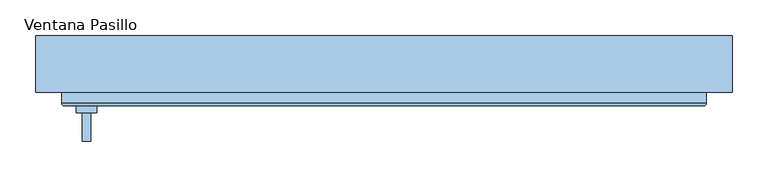
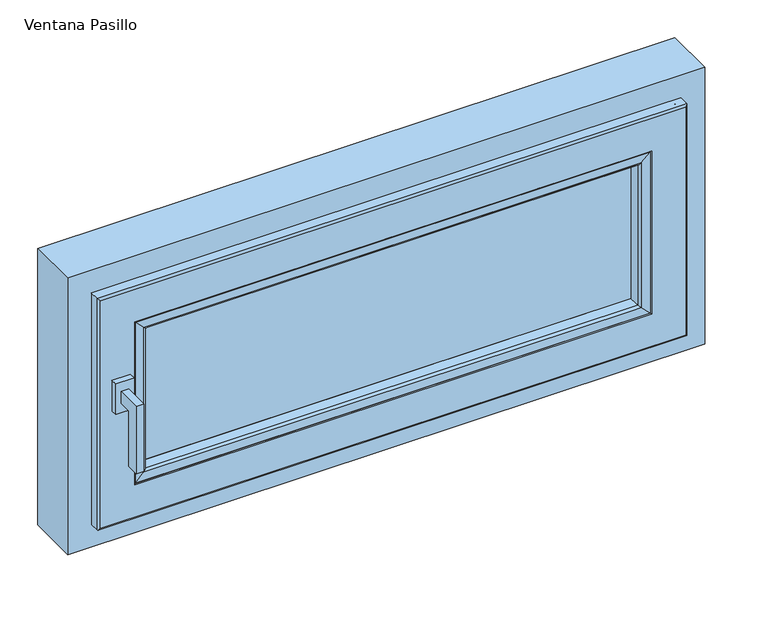
"""IFC4 building model written with IfcOpenShell, lengths in millimetres: window geometry, 2019_ES_Ventana_Replus_re80pvc301_10100_1-Hoja : Ventana Pasillo."""

from ifc_helpers import new_model, si_unit, frame, origin, place, context, project, spatial, polyline, ellipse_curve, outline, extrude, source, transform, mapped, element, save
from ifc_brep_helpers import plane_surface, cylinder_surface, advanced_brep


def ventana_pasillo_7f72e0b0(model_context):
    return source(origin(), model_context, "Body", "SolidModel", [
        extrude(outline(polyline([(-78.4999991, 1070.0), (-78.4999991, 1050.0), (-98.4999991, 1050.0), (-98.4999991, 960.0), (-118.4999991, 960.0), (-118.4999991, 1070.0), (-78.4999991, 1070.0)])), frame((-424.1999993, 0.0, 0.0), z_axis=(1.0, 0.0, 0.0), x_axis=(0.0, 1.0, 0.0)), (0.0, 0.0, 1.0), 12.0),
        extrude(outline(polyline([(-403.9687607, -78.4999991), (-432.4312378, -78.4999991), (-432.4312378, -68.4999991), (-403.9687607, -68.4999991), (-403.9687607, -78.4999991)])), frame((0.0, 0.0, 1035.217127), z_axis=(0.0, 0.0, 1.0), x_axis=(1.0, 0.0, 0.0)), (0.0, 0.0, 1.0), 49.565746),
        extrude(outline(polyline([(1157.2, 387.1999993), (1157.2, -387.1999993), (909.8, -387.1999993), (909.8, 387.1999993), (1157.2, 387.1999993)]), holes=[polyline([(917.8, 379.1999993), (917.8, -379.1999993), (1149.2, -379.1999993), (1149.2, 379.1999993), (917.8, 379.1999993)])]), frame((0.0, -26.9999999, 0.0), z_axis=(0.0, 1.0, 0.0), x_axis=(0.0, 0.0, 1.0)), (0.0, 0.0, 1.0), 16.0),
        extrude(outline(polyline([(1157.1868066, 387.1868058), (1157.1868066, -387.1868058), (909.8131934, -387.1868058), (909.8131934, 387.1868058), (1157.1868066, 387.1868058)]), holes=[polyline([(917.8, 379.1999993), (917.8, -379.1999993), (1149.2, -379.1999993), (1149.2, 379.1999993), (917.8, 379.1999993)])]), frame((0.0, -47.0000001, 0.0), z_axis=(0.0, 1.0, 0.0), x_axis=(0.0, 0.0, 1.0)), (0.0, 0.0, 1.0), 16.0),
        extrude(outline(polyline([(387.1999993, -6.9999997), (387.1999993, -10.9999999), (-387.1999993, -10.9999999), (-387.1999993, -6.9999997), (387.1999993, -6.9999997)])), frame((0.0, 0.0, 903.7946451), z_axis=(0.0, 0.0, 1.0), x_axis=(1.0, 0.0, 0.0)), (0.0, 0.0, 1.0), 259.4053549),
        extrude(outline(polyline([(387.1999993, -26.9999999), (387.1999993, -31.0000001), (-387.1999993, -31.0000001), (-387.1999993, -26.9999999), (387.1999993, -26.9999999)])), frame((0.0, 0.0, 903.7946451), z_axis=(0.0, 0.0, 1.0), x_axis=(1.0, 0.0, 0.0)), (0.0, 0.0, 1.0), 259.4053549),
        extrude(outline(polyline([(387.1999993, -47.0000001), (387.1999993, -51.0000003), (-387.1999993, -51.0000003), (-387.1999993, -47.0000001), (387.1999993, -47.0000001)])), frame((0.0, 0.0, 903.7946451), z_axis=(0.0, 0.0, 1.0), x_axis=(1.0, 0.0, 0.0)), (0.0, 0.0, 1.0), 259.4053549),
        advanced_brep(
        [(377.2913171, 9.2764571, 1147.2913178), (380.1890946, 11.5, 1150.1890953), (380.1890946, 11.5, 919.8109047), (377.2913171, 9.2764571, 922.7086822), (420.1999993, 11.5, 879.8), (-420.1999993, 11.5, 879.8), (-420.1999993, 11.5, 1190.2), (420.1999993, 11.5, 1190.2), (-380.1890946, 11.5, 1150.1890953), (-380.1890946, 11.5, 919.8109047), (-377.2913171, 9.2764571, 922.7086822), (374.1757968, -2.3508228, 1144.1757976), (374.1757968, -2.3508228, 925.8242024), (-374.1757968, -2.3508228, 925.8242024), (374.6739305, -3.0000033, 1144.6739313), (374.6739305, -3.0000033, 925.3260687), (-374.6739305, -3.0000033, 925.3260687), (381.1999993, -3.0000033, 1151.2), (-381.1999993, -3.0000033, 1151.2), (-381.1999993, -3.0000033, 918.8), (381.1999993, -3.0000033, 918.8), (-374.6739305, -3.0000033, 1144.6739313), (381.1999993, -6.9999997, 1151.2), (381.1999993, -6.9999997, 918.8), (-381.1999993, -6.9999997, 918.8), (401.8162192, -6.9999997, 1171.8162199), (-401.8162192, -6.9999997, 1171.8162199), (-401.8162192, -6.9999997, 898.1837801), (401.8162192, -6.9999997, 898.1837801), (-381.1999993, -6.9999997, 1151.2), (399.1999993, -25.6153717, 1169.2), (399.1999993, -25.6153717, 900.8), (-399.1999993, -25.6153717, 900.8), (399.1999993, -56.4999995, 1169.2), (399.1999993, -56.4999995, 900.8), (-399.1999993, -56.4999995, 900.8), (-399.1999993, -56.4999995, 1169.2), (387.1999993, -56.4999995, 1157.2), (-387.1999993, -56.4999995, 1157.2), (-387.1999993, -56.4999995, 912.8), (387.1999993, -56.4999995, 912.8), (387.1999993, -51.0000003, 1157.2), (387.1999993, -51.0000003, 912.8), (-387.1999993, -51.0000003, 912.8), (-387.1999993, -51.0000003, 1157.2), (376.007687, -51.0000003, 1146.0076877), (-376.007687, -51.0000003, 1146.0076877), (-376.007687, -51.0000003, 923.9923123), (376.007687, -51.0000003, 923.9923123), (375.4940999, -51.6693201, 1145.4941006), (375.4940999, -51.6693201, 924.5058994), (-375.4940999, -51.6693201, 924.5058994), (378.8993918, -64.3780426, 1148.8993925), (378.8993918, -64.3780426, 921.1006075), (-378.8993918, -64.3780426, 921.1006075), (382.6234971, -67.3403297, 1152.6234978), (382.6234971, -67.3403297, 917.3765022), (-382.6234971, -67.3403297, 917.3765022), (395.6488427, -67.7951848, 1165.6488434), (395.6488427, -67.7951848, 904.3511566), (-395.6488427, -67.7951848, 904.3511566), (396.1999993, -67.2629391, 1166.2), (396.1999993, -67.2629391, 903.8), (-396.1999993, -67.2629391, 903.8), (397.4370593, -68.4999991, 1167.43706), (397.4370593, -68.4999991, 902.56294), (-397.4370593, -68.4999991, 902.56294), (450.1999993, -68.4999991, 1220.2), (-450.1999993, -68.4999991, 1220.2), (-450.1999993, -68.4999991, 849.8), (450.1999993, -68.4999991, 849.8), (-397.4370593, -68.4999991, 1167.43706), (453.1999993, -65.4999991, 1223.2), (453.1999993, -65.4999991, 846.8), (-453.1999993, -65.4999991, 846.8), (453.1999993, -50.0, 1223.2), (453.1999993, -50.0, 846.8), (-453.1999993, -50.0, 846.8), (-453.1999993, -50.0, 1223.2), (433.1999993, -50.0, 1203.2), (-433.1999993, -50.0, 1203.2), (-433.1999993, -50.0, 866.8), (433.1999993, -50.0, 866.8), (433.1999993, -11.9999991, 866.8), (433.1999993, -11.9999991, 1203.2), (-433.1999993, -11.9999991, 866.8), (-433.1999993, -11.9999991, 1203.2), (420.1999993, -11.9999991, 1190.2), (-420.1999993, -11.9999991, 1190.2), (-420.1999993, -11.9999991, 879.8), (420.1999993, -11.9999991, 879.8), (-377.2913171, 9.2764571, 1147.2913178), (-374.1757968, -2.3508228, 1144.1757976), (-399.1999993, -25.6153717, 1169.2), (-375.4940999, -51.6693201, 1145.4941006), (-378.8993918, -64.3780426, 1148.8993925), (-382.6234971, -67.3403297, 1152.6234978), (-395.6488427, -67.7951848, 1165.6488434), (-396.1999993, -67.2629391, 1166.2), (-453.1999993, -65.4999991, 1223.2)],
        [
            (0, 1, ellipse_curve(frame((380.1890946, 8.5, 1150.1890953), z_axis=(0.7071067811865475, 0.0, -0.7071067811865475), x_axis=(0.7071067811865474, 0.0, 0.7071067811865476)), 4.2426407, 3.0)),
            (1, 2),
            (2, 3, ellipse_curve(frame((380.1890946, 8.5, 919.8109047), z_axis=(0.7071067811865475, 0.0, 0.7071067811865475), x_axis=(-0.7071067811865474, 0.0, 0.7071067811865476)), 4.2426407, 3.0)),
            (3, 0),
            (4, 5),
            (5, 6),
            (6, 7),
            (7, 4),
            (1, 8),
            (8, 9),
            (9, 2),
            (9, 10, ellipse_curve(frame((-380.1890946, 8.5, 919.8109047), z_axis=(0.7071067811865475, 0.0, -0.7071067811865475), x_axis=(0.7071067811865476, 0.0, 0.7071067811865474)), 4.2426407, 3.0)),
            (10, 3),
            (11, 0),
            (3, 12),
            (12, 11),
            (10, 13),
            (13, 12),
            (14, 11, ellipse_curve(frame((374.6739305, -2.4842973, 1144.6739313), z_axis=(0.7071067811865475, 0.0, -0.7071067811865475), x_axis=(0.7071067811865474, 0.0, 0.7071067811865476)), 0.7293184, 0.515706)),
            (12, 15, ellipse_curve(frame((374.6739305, -2.4842973, 925.3260687), z_axis=(0.7071067811865475, 0.0, 0.7071067811865475), x_axis=(-0.7071067811865474, 0.0, 0.7071067811865476)), 0.7293184, 0.515706)),
            (15, 14),
            (13, 16, ellipse_curve(frame((-374.6739305, -2.4842973, 925.3260687), z_axis=(0.7071067811865475, 0.0, -0.7071067811865475), x_axis=(0.7071067811865476, 0.0, 0.7071067811865474)), 0.7293184, 0.515706)),
            (16, 15),
            (17, 18),
            (18, 19),
            (19, 20),
            (20, 17),
            (16, 21),
            (21, 14),
            (22, 17),
            (20, 23),
            (23, 22),
            (19, 24),
            (24, 23),
            (25, 26),
            (26, 27),
            (27, 28),
            (28, 25),
            (24, 29),
            (29, 22),
            (30, 25),
            (28, 31),
            (31, 30),
            (27, 32),
            (32, 31),
            (33, 30),
            (31, 34),
            (34, 33),
            (32, 35),
            (35, 34),
            (35, 36),
            (36, 33),
            (37, 38),
            (38, 39),
            (39, 40),
            (40, 37),
            (41, 37),
            (40, 42),
            (42, 41),
            (39, 43),
            (43, 42),
            (43, 44),
            (44, 41),
            (45, 46),
            (46, 47),
            (47, 48),
            (48, 45),
            (49, 45, ellipse_curve(frame((376.007687, -51.5317048, 1146.0076877), z_axis=(0.7071067811865475, 0.0, -0.7071067811865475), x_axis=(0.7071067811865474, 0.0, 0.7071067811865476)), 0.7519437, 0.5317045)),
            (48, 50, ellipse_curve(frame((376.007687, -51.5317048, 923.9923123), z_axis=(0.7071067811865475, 0.0, 0.7071067811865475), x_axis=(-0.7071067811865474, 0.0, 0.7071067811865476)), 0.7519437, 0.5317045)),
            (50, 49),
            (47, 51, ellipse_curve(frame((-376.007687, -51.5317048, 923.9923123), z_axis=(0.7071067811865475, 0.0, -0.7071067811865475), x_axis=(0.7071067811865476, 0.0, 0.7071067811865474)), 0.7519437, 0.5317045)),
            (51, 50),
            (52, 49),
            (50, 53),
            (53, 52),
            (51, 54),
            (54, 53),
            (55, 52, ellipse_curve(frame((382.7630951, -63.3427664, 1152.7630958), z_axis=(0.7071067811865475, 0.0, -0.7071067811865475), x_axis=(0.7071067811865474, 0.0, 0.7071067811865476)), 5.6568542, 4.0)),
            (53, 56, ellipse_curve(frame((382.7630951, -63.3427664, 917.2369042), z_axis=(0.7071067811865475, 0.0, 0.7071067811865475), x_axis=(-0.7071067811865474, 0.0, 0.7071067811865476)), 5.6568542, 4.0)),
            (56, 55),
            (54, 57, ellipse_curve(frame((-382.7630951, -63.3427664, 917.2369042), z_axis=(0.7071067811865475, 0.0, -0.7071067811865475), x_axis=(0.7071067811865476, 0.0, 0.7071067811865474)), 5.6568542, 4.0)),
            (57, 56),
            (58, 55),
            (56, 59),
            (59, 58),
            (57, 60),
            (60, 59),
            (61, 58, ellipse_curve(frame((395.6674291, -67.2629391, 1165.6674299), z_axis=(0.7071067811865475, 0.0, -0.7071067811865475), x_axis=(0.7071067811865474, 0.0, 0.7071067811865476)), 0.7531679, 0.5325701)),
            (59, 62, ellipse_curve(frame((395.6674291, -67.2629391, 904.3325701), z_axis=(0.7071067811865475, 0.0, 0.7071067811865475), x_axis=(-0.7071067811865474, 0.0, 0.7071067811865476)), 0.7531679, 0.5325701)),
            (62, 61),
            (60, 63, ellipse_curve(frame((-395.6674291, -67.2629391, 904.3325701), z_axis=(0.7071067811865475, 0.0, -0.7071067811865475), x_axis=(0.7071067811865476, 0.0, 0.7071067811865474)), 0.7531679, 0.5325701)),
            (63, 62),
            (64, 61, ellipse_curve(frame((397.4370593, -67.2629391, 1167.43706), z_axis=(0.7071067811865475, 0.0, -0.7071067811865475), x_axis=(0.7071067811865474, 0.0, 0.7071067811865476)), 1.7494671, 1.23706)),
            (62, 65, ellipse_curve(frame((397.4370593, -67.2629391, 902.56294), z_axis=(0.7071067811865475, 0.0, 0.7071067811865475), x_axis=(-0.7071067811865474, 0.0, 0.7071067811865476)), 1.7494671, 1.23706)),
            (65, 64),
            (63, 66, ellipse_curve(frame((-397.4370593, -67.2629391, 902.56294), z_axis=(0.7071067811865475, 0.0, -0.7071067811865475), x_axis=(0.7071067811865476, 0.0, 0.7071067811865474)), 1.7494671, 1.23706)),
            (66, 65),
            (67, 68),
            (68, 69),
            (69, 70),
            (70, 67),
            (66, 71),
            (71, 64),
            (72, 67, ellipse_curve(frame((450.1999993, -65.4999991, 1220.2), z_axis=(0.7071067811865475, 0.0, -0.7071067811865475), x_axis=(0.7071067811865474, 0.0, 0.7071067811865476)), 4.2426407, 3.0)),
            (70, 73, ellipse_curve(frame((450.1999993, -65.4999991, 849.8), z_axis=(0.7071067811865475, 0.0, 0.7071067811865475), x_axis=(-0.7071067811865474, 0.0, 0.7071067811865476)), 4.2426407, 3.0)),
            (73, 72),
            (69, 74, ellipse_curve(frame((-450.1999993, -65.4999991, 849.8), z_axis=(0.7071067811865475, 0.0, -0.7071067811865475), x_axis=(0.7071067811865476, 0.0, 0.7071067811865474)), 4.2426407, 3.0)),
            (74, 73),
            (75, 72),
            (73, 76),
            (76, 75),
            (74, 77),
            (77, 76),
            (77, 78),
            (78, 75),
            (79, 80),
            (80, 81),
            (81, 82),
            (82, 79),
            (82, 83),
            (83, 84),
            (84, 79),
            (81, 85),
            (85, 83),
            (85, 86),
            (86, 84),
            (87, 88),
            (88, 89),
            (89, 90),
            (90, 87),
            (90, 4),
            (7, 87),
            (89, 5),
            (8, 91, ellipse_curve(frame((-380.1890946, 8.5, 1150.1890953), z_axis=(-0.7071067811865475, 0.0, -0.7071067811865475), x_axis=(0.7071067811865474, 0.0, -0.7071067811865476)), 4.2426407, 3.0)),
            (91, 10),
            (91, 92),
            (92, 13),
            (92, 21, ellipse_curve(frame((-374.6739305, -2.4842973, 1144.6739313), z_axis=(-0.7071067811865475, 0.0, -0.7071067811865475), x_axis=(0.7071067811865474, 0.0, -0.7071067811865476)), 0.7293184, 0.515706)),
            (18, 29),
            (26, 93),
            (93, 32),
            (93, 36),
            (38, 44),
            (46, 94, ellipse_curve(frame((-376.007687, -51.5317048, 1146.0076877), z_axis=(-0.7071067811865475, 0.0, -0.7071067811865475), x_axis=(0.7071067811865474, 0.0, -0.7071067811865476)), 0.7519437, 0.5317045)),
            (94, 51),
            (94, 95),
            (95, 54),
            (95, 96, ellipse_curve(frame((-382.7630951, -63.3427664, 1152.7630958), z_axis=(-0.7071067811865475, 0.0, -0.7071067811865475), x_axis=(0.7071067811865474, 0.0, -0.7071067811865476)), 5.6568542, 4.0)),
            (96, 57),
            (96, 97),
            (97, 60),
            (97, 98, ellipse_curve(frame((-395.6674291, -67.2629391, 1165.6674299), z_axis=(-0.7071067811865475, 0.0, -0.7071067811865475), x_axis=(0.7071067811865474, 0.0, -0.7071067811865476)), 0.7531679, 0.5325701)),
            (98, 63),
            (98, 71, ellipse_curve(frame((-397.4370593, -67.2629391, 1167.43706), z_axis=(-0.7071067811865475, 0.0, -0.7071067811865475), x_axis=(0.7071067811865474, 0.0, -0.7071067811865476)), 1.7494671, 1.23706)),
            (68, 99, ellipse_curve(frame((-450.1999993, -65.4999991, 1220.2), z_axis=(-0.7071067811865475, 0.0, -0.7071067811865475), x_axis=(0.7071067811865474, 0.0, -0.7071067811865476)), 4.2426407, 3.0)),
            (99, 74),
            (99, 78),
            (80, 86),
            (88, 6),
            (0, 91),
            (11, 92),
            (30, 93),
            (49, 94),
            (52, 95),
            (55, 96),
            (58, 97),
            (61, 98),
            (72, 99),
        ],
        [
            cylinder_surface(frame((380.1890946, 8.5, 1223.2), z_axis=(0.0, 0.0, 1.0), x_axis=(-1.0, 0.0, 0.0)), 3.0),
            plane_surface(frame((-420.1999993, 11.5, 1190.2), z_axis=(0.0, 1.0, 0.0), x_axis=(1.0, 0.0, 0.0))),
            cylinder_surface(frame((453.1999993, 8.5, 919.8109047), z_axis=(1.0, 0.0, 0.0), x_axis=(0.0, 0.0, 1.0)), 3.0),
            plane_surface(frame((377.2913171, 9.2764571, 1147.2913178), z_axis=(-0.9659258263570549, 0.25881904484879154, 0.0), x_axis=(0.0, 0.0, -1.0))),
            plane_surface(frame((377.2913171, 9.2764571, 922.7086822), z_axis=(0.0, 0.2588190448487884, 0.9659258263570558), x_axis=(-1.0, 0.0, 0.0))),
            cylinder_surface(frame((374.6739305, -2.4842973, 1223.2), z_axis=(0.0, 0.0, 1.0), x_axis=(-1.0, 0.0, 0.0)), 0.515706),
            cylinder_surface(frame((453.1999993, -2.4842973, 925.3260687), z_axis=(1.0, 0.0, 0.0), x_axis=(0.0, 0.0, 1.0)), 0.515706),
            plane_surface(frame((-374.6739305, -3.0000033, 1144.6739313), z_axis=(0.0, -1.0, 0.0), x_axis=(1.0, 0.0, 0.0))),
            plane_surface(frame((381.1999993, -3.0000033, 1151.2), z_axis=(-1.0, 0.0, 0.0), x_axis=(0.0, 0.0, -1.0))),
            plane_surface(frame((381.1999993, -3.0000033, 918.8), z_axis=(0.0, 0.0, 1.0), x_axis=(-1.0, 0.0, 0.0))),
            plane_surface(frame((-381.1999993, -6.9999997, 1151.2), z_axis=(0.0, -1.0, 0.0), x_axis=(1.0, 0.0, 0.0))),
            plane_surface(frame((401.8162192, -6.9999997, 1171.8162199), z_axis=(-0.9902680687415736, 0.13917310096004262, 0.0), x_axis=(0.0, 0.0, -1.0))),
            plane_surface(frame((401.8162192, -6.9999997, 898.1837801), z_axis=(0.0, 0.13917310096003943, 0.990268068741574), x_axis=(-1.0, 0.0, 0.0))),
            plane_surface(frame((399.1999993, -25.6153717, 1169.2), z_axis=(-1.0, 0.0, 0.0), x_axis=(0.0, 0.0, -1.0))),
            plane_surface(frame((399.1999993, -25.6153717, 900.8), z_axis=(0.0, 0.0, 1.0), x_axis=(-1.0, 0.0, 0.0))),
            plane_surface(frame((-399.1999993, -56.4999995, 1169.2), z_axis=(0.0, 1.0, 0.0), x_axis=(1.0, 0.0, 0.0))),
            plane_surface(frame((387.1999993, -56.4999995, 1157.2), z_axis=(1.0, 0.0, 0.0), x_axis=(0.0, 0.0, -1.0))),
            plane_surface(frame((387.1999993, -56.4999995, 912.8), z_axis=(0.0, 0.0, -1.0), x_axis=(-1.0, 0.0, 0.0))),
            plane_surface(frame((-387.1999993, -51.0000003, 1157.2), z_axis=(0.0, 1.0, 0.0), x_axis=(1.0, 0.0, 0.0))),
            cylinder_surface(frame((376.007687, -51.5317048, 1223.2), z_axis=(0.0, 0.0, 1.0), x_axis=(-1.0, 0.0, 0.0)), 0.5317045),
            cylinder_surface(frame((453.1999993, -51.5317048, 923.9923123), z_axis=(1.0, 0.0, 0.0), x_axis=(0.0, 0.0, 1.0)), 0.5317045),
            plane_surface(frame((375.4940999, -51.6693201, 1145.4941006), z_axis=(-0.9659258262890666, -0.25881904510252723, 0.0), x_axis=(0.0, 0.0, -1.0))),
            plane_surface(frame((375.4940999, -51.6693201, 924.5058994), z_axis=(0.0, -0.25881904510253034, 0.9659258262890658), x_axis=(-1.0, 0.0, 0.0))),
            cylinder_surface(frame((382.7630951, -63.3427664, 1223.2), z_axis=(0.0, 0.0, 1.0), x_axis=(-1.0, 0.0, 0.0)), 4.0),
            cylinder_surface(frame((453.1999993, -63.3427664, 917.2369042), z_axis=(1.0, 0.0, 0.0), x_axis=(0.0, 0.0, 1.0)), 4.0),
            plane_surface(frame((382.6234971, -67.3403297, 1152.6234978), z_axis=(-0.0348994967025078, -0.9993908270190955, 0.0), x_axis=(0.0, 0.0, -1.0))),
            plane_surface(frame((382.6234971, -67.3403297, 917.3765022), z_axis=(0.0, -0.9993908270190957, 0.03489949670250457), x_axis=(-1.0, 0.0, 0.0))),
            cylinder_surface(frame((395.6674291, -67.2629391, 1223.2), z_axis=(0.0, 0.0, 1.0), x_axis=(-1.0, 0.0, 0.0)), 0.5325701),
            cylinder_surface(frame((453.1999993, -67.2629391, 904.3325701), z_axis=(1.0, 0.0, 0.0), x_axis=(0.0, 0.0, 1.0)), 0.5325701),
            cylinder_surface(frame((397.4370593, -67.2629391, 1223.2), z_axis=(0.0, 0.0, 1.0), x_axis=(-1.0, 0.0, 0.0)), 1.23706),
            cylinder_surface(frame((453.1999993, -67.2629391, 902.56294), z_axis=(1.0, 0.0, 0.0), x_axis=(0.0, 0.0, 1.0)), 1.23706),
            plane_surface(frame((-397.4370593, -68.4999991, 1167.43706), z_axis=(0.0, -1.0, 0.0), x_axis=(1.0, 0.0, 0.0))),
            cylinder_surface(frame((450.1999993, -65.4999991, 1223.2), z_axis=(0.0, 0.0, 1.0), x_axis=(-1.0, 0.0, 0.0)), 3.0),
            cylinder_surface(frame((453.1999993, -65.4999991, 849.8), z_axis=(1.0, 0.0, 0.0), x_axis=(0.0, 0.0, 1.0)), 3.0),
            plane_surface(frame((453.1999993, -65.4999991, 1223.2), z_axis=(1.0, 0.0, 0.0), x_axis=(0.0, 0.0, -1.0))),
            plane_surface(frame((453.1999993, -65.4999991, 846.8), z_axis=(0.0, 0.0, -1.0), x_axis=(-1.0, 0.0, 0.0))),
            plane_surface(frame((-449.2000019, -50.0, 1219.2000027), z_axis=(0.0, 1.0, 0.0), x_axis=(1.0, 0.0, 0.0))),
            plane_surface(frame((433.1999993, -45.0999991, 1203.2), z_axis=(1.0, 0.0, 0.0), x_axis=(0.0, 0.0, -1.0))),
            plane_surface(frame((433.1999993, -45.0999991, 866.8), z_axis=(0.0, 0.0, -1.0), x_axis=(-1.0, 0.0, 0.0))),
            plane_surface(frame((-425.7000002, -11.9999991, 1195.7000009), z_axis=(0.0, 1.0, 0.0), x_axis=(1.0, 0.0, 0.0))),
            plane_surface(frame((420.1999993, -1.4999991, 1190.2), z_axis=(1.0, 0.0, 0.0), x_axis=(0.0, 0.0, -1.0))),
            plane_surface(frame((420.1999993, -1.4999991, 879.8), z_axis=(0.0, 0.0, -1.0), x_axis=(-1.0, 0.0, 0.0))),
            cylinder_surface(frame((-380.1890946, 8.5, 846.8), z_axis=(0.0, 0.0, -1.0), x_axis=(1.0, 0.0, 0.0)), 3.0),
            plane_surface(frame((-377.2913171, 9.2764571, 922.7086822), z_axis=(0.9659258263570565, 0.25881904484878526, 0.0), x_axis=(0.0, 0.0, 1.0))),
            cylinder_surface(frame((-374.6739305, -2.4842973, 846.8), z_axis=(0.0, 0.0, -1.0), x_axis=(1.0, 0.0, 0.0)), 0.515706),
            plane_surface(frame((-381.1999993, -3.0000033, 918.8), z_axis=(1.0, 0.0, 0.0), x_axis=(0.0, 0.0, 1.0))),
            plane_surface(frame((-401.8162192, -6.9999997, 898.1837801), z_axis=(0.9902680687415745, 0.13917310096003624, 0.0), x_axis=(0.0, 0.0, 1.0))),
            plane_surface(frame((-399.1999993, -25.6153717, 900.8), z_axis=(1.0, 0.0, 0.0), x_axis=(0.0, 0.0, 1.0))),
            plane_surface(frame((-387.1999993, -56.4999995, 912.8), z_axis=(-1.0, 0.0, 0.0), x_axis=(0.0, 0.0, 1.0))),
            cylinder_surface(frame((-376.007687, -51.5317048, 846.8), z_axis=(0.0, 0.0, -1.0), x_axis=(1.0, 0.0, 0.0)), 0.5317045),
            plane_surface(frame((-375.4940999, -51.6693201, 924.5058994), z_axis=(0.9659258262890649, -0.25881904510253345, 0.0), x_axis=(0.0, 0.0, 1.0))),
            cylinder_surface(frame((-382.7630951, -63.3427664, 846.8), z_axis=(0.0, 0.0, -1.0), x_axis=(1.0, 0.0, 0.0)), 4.0),
            plane_surface(frame((-382.6234971, -67.3403297, 917.3765022), z_axis=(0.034899496702501344, -0.9993908270190958, 0.0), x_axis=(0.0, 0.0, 1.0))),
            cylinder_surface(frame((-395.6674291, -67.2629391, 846.8), z_axis=(0.0, 0.0, -1.0), x_axis=(1.0, 0.0, 0.0)), 0.5325701),
            cylinder_surface(frame((-397.4370593, -67.2629391, 846.8), z_axis=(0.0, 0.0, -1.0), x_axis=(1.0, 0.0, 0.0)), 1.23706),
            cylinder_surface(frame((-450.1999993, -65.4999991, 846.8), z_axis=(0.0, 0.0, -1.0), x_axis=(1.0, 0.0, 0.0)), 3.0),
            plane_surface(frame((-453.1999993, -65.4999991, 846.8), z_axis=(-1.0, 0.0, 0.0), x_axis=(0.0, 0.0, 1.0))),
            plane_surface(frame((-433.1999993, -45.0999991, 866.8), z_axis=(-1.0, 0.0, 0.0), x_axis=(0.0, 0.0, 1.0))),
            plane_surface(frame((-420.1999993, -1.4999991, 879.8), z_axis=(-1.0, 0.0, 0.0), x_axis=(0.0, 0.0, 1.0))),
            cylinder_surface(frame((-453.1999993, 8.5, 1150.1890953), z_axis=(-1.0, 0.0, 0.0), x_axis=(0.0, 0.0, -1.0)), 3.0),
            plane_surface(frame((-377.2913171, 9.2764571, 1147.2913178), z_axis=(0.0, 0.2588190448487884, -0.9659258263570557), x_axis=(1.0, 0.0, 0.0))),
            cylinder_surface(frame((-453.1999993, -2.4842973, 1144.6739313), z_axis=(-1.0, 0.0, 0.0), x_axis=(0.0, 0.0, -1.0)), 0.515706),
            plane_surface(frame((-381.1999993, -3.0000033, 1151.2), z_axis=(0.0, 0.0, -1.0), x_axis=(1.0, 0.0, 0.0))),
            plane_surface(frame((-401.8162192, -6.9999997, 1171.8162199), z_axis=(0.0, 0.13917310096003943, -0.990268068741574), x_axis=(1.0, 0.0, 0.0))),
            plane_surface(frame((-399.1999993, -25.6153717, 1169.2), z_axis=(0.0, 0.0, -1.0), x_axis=(1.0, 0.0, 0.0))),
            plane_surface(frame((-387.1999993, -56.4999995, 1157.2), z_axis=(0.0, 0.0, 1.0), x_axis=(1.0, 0.0, 0.0))),
            cylinder_surface(frame((-453.1999993, -51.5317048, 1146.0076877), z_axis=(-1.0, 0.0, 0.0), x_axis=(0.0, 0.0, -1.0)), 0.5317045),
            plane_surface(frame((-375.4940999, -51.6693201, 1145.4941006), z_axis=(0.0, -0.25881904510253034, -0.9659258262890658), x_axis=(1.0, 0.0, 0.0))),
            cylinder_surface(frame((-453.1999993, -63.3427664, 1152.7630958), z_axis=(-1.0, 0.0, 0.0), x_axis=(0.0, 0.0, -1.0)), 4.0),
            plane_surface(frame((-382.6234971, -67.3403297, 1152.6234978), z_axis=(0.0, -0.9993908270190957, -0.03489949670250457), x_axis=(1.0, 0.0, 0.0))),
            cylinder_surface(frame((-453.1999993, -67.2629391, 1165.6674299), z_axis=(-1.0, 0.0, 0.0), x_axis=(0.0, 0.0, -1.0)), 0.5325701),
            cylinder_surface(frame((-453.1999993, -67.2629391, 1167.43706), z_axis=(-1.0, 0.0, 0.0), x_axis=(0.0, 0.0, -1.0)), 1.23706),
            cylinder_surface(frame((-453.1999993, -65.4999991, 1220.2), z_axis=(-1.0, 0.0, 0.0), x_axis=(0.0, 0.0, -1.0)), 3.0),
            plane_surface(frame((-453.1999993, -65.4999991, 1223.2), z_axis=(0.0, 0.0, 1.0), x_axis=(1.0, 0.0, 0.0))),
            plane_surface(frame((-433.1999993, -45.0999991, 1203.2), z_axis=(0.0, 0.0, 1.0), x_axis=(1.0, 0.0, 0.0))),
            plane_surface(frame((-420.1999993, -1.4999991, 1190.2), z_axis=(0.0, 0.0, 1.0), x_axis=(1.0, 0.0, 0.0))),
        ],
        [
            (0, [[1, 2, 3, 4]]),
            (1, [[5, 6, 7, 8], [9, 10, 11, -2]]),
            (2, [[-3, -11, 12, 13]]),
            (3, [[14, -4, 15, 16]]),
            (4, [[-15, -13, 17, 18]]),
            (5, [[19, -16, 20, 21]]),
            (6, [[-20, -18, 22, 23]]),
            (7, [[24, 25, 26, 27], [-23, 28, 29, -21]]),
            (8, [[30, -27, 31, 32]]),
            (9, [[-31, -26, 33, 34]]),
            (10, [[35, 36, 37, 38], [-34, 39, 40, -32]]),
            (11, [[41, -38, 42, 43]]),
            (12, [[-42, -37, 44, 45]]),
            (13, [[46, -43, 47, 48]]),
            (14, [[-47, -45, 49, 50]]),
            (15, [[-50, 51, 52, -48], [53, 54, 55, 56]]),
            (16, [[57, -56, 58, 59]]),
            (17, [[-58, -55, 60, 61]]),
            (18, [[-61, 62, 63, -59], [64, 65, 66, 67]]),
            (19, [[68, -67, 69, 70]]),
            (20, [[-69, -66, 71, 72]]),
            (21, [[73, -70, 74, 75]]),
            (22, [[-74, -72, 76, 77]]),
            (23, [[78, -75, 79, 80]]),
            (24, [[-79, -77, 81, 82]]),
            (25, [[83, -80, 84, 85]]),
            (26, [[-84, -82, 86, 87]]),
            (27, [[88, -85, 89, 90]]),
            (28, [[-89, -87, 91, 92]]),
            (29, [[93, -90, 94, 95]]),
            (30, [[-94, -92, 96, 97]]),
            (31, [[98, 99, 100, 101], [-97, 102, 103, -95]]),
            (32, [[104, -101, 105, 106]]),
            (33, [[-105, -100, 107, 108]]),
            (34, [[109, -106, 110, 111]]),
            (35, [[-110, -108, 112, 113]]),
            (36, [[-113, 114, 115, -111], [116, 117, 118, 119]]),
            (37, [[-119, 120, 121, 122]]),
            (38, [[-120, -118, 123, 124]]),
            (39, [[-124, 125, 126, -121], [127, 128, 129, 130]]),
            (40, [[-130, 131, -8, 132]]),
            (41, [[-131, -129, 133, -5]]),
            (42, [[-12, -10, 134, 135]]),
            (43, [[-17, -135, 136, 137]]),
            (44, [[-22, -137, 138, -28]]),
            (45, [[-33, -25, 139, -39]]),
            (46, [[-44, -36, 140, 141]]),
            (47, [[-49, -141, 142, -51]]),
            (48, [[-60, -54, 143, -62]]),
            (49, [[-71, -65, 144, 145]]),
            (50, [[-76, -145, 146, 147]]),
            (51, [[-81, -147, 148, 149]]),
            (52, [[-86, -149, 150, 151]]),
            (53, [[-91, -151, 152, 153]]),
            (54, [[-96, -153, 154, -102]]),
            (55, [[-107, -99, 155, 156]]),
            (56, [[-112, -156, 157, -114]]),
            (57, [[-123, -117, 158, -125]]),
            (58, [[-133, -128, 159, -6]]),
            (59, [[-134, -9, -1, 160]]),
            (60, [[-136, -160, -14, 161]]),
            (61, [[-138, -161, -19, -29]]),
            (62, [[-139, -24, -30, -40]]),
            (63, [[-140, -35, -41, 162]]),
            (64, [[-142, -162, -46, -52]]),
            (65, [[-143, -53, -57, -63]]),
            (66, [[-144, -64, -68, 163]]),
            (67, [[-146, -163, -73, 164]]),
            (68, [[-148, -164, -78, 165]]),
            (69, [[-150, -165, -83, 166]]),
            (70, [[-152, -166, -88, 167]]),
            (71, [[-154, -167, -93, -103]]),
            (72, [[-155, -98, -104, 168]]),
            (73, [[-157, -168, -109, -115]]),
            (74, [[-158, -116, -122, -126]]),
            (75, [[-159, -127, -132, -7]]),
        ],
    ),
        advanced_brep(
        [(413.2673545, 12.758819, 1183.2673545), (417.2913185, 27.7764571, 1187.2913185), (417.2913185, 27.7764571, 882.7086815), (413.2673545, 12.758819, 886.7326455), (420.189096, 30.0, 1190.189096), (420.189096, 30.0, 879.810904), (-417.2913185, 27.7764571, 882.7086815), (-413.2673545, 12.758819, 886.7326455), (414.2332803, 11.5, 1184.2332803), (414.2332803, 11.5, 885.7667197), (490.0, 30.0, 1260.0), (490.0, -50.0, 1260.0), (490.0, -50.0, 810.0), (490.0, 30.0, 810.0), (-490.0, -50.0, 1260.0), (-490.0, -50.0, 810.0), (446.1999993, -50.0, 853.8000007), (-446.1999993, -50.0, 853.8000007), (-446.1999993, -50.0, 1216.1999993), (446.1999993, -50.0, 1216.1999993), (-490.0, 30.0, 810.0), (-490.0, 30.0, 1260.0), (-420.189096, 30.0, 1190.189096), (-420.189096, 30.0, 879.810904), (426.1891471, -8.0, 1196.1891471), (426.1891471, 11.5, 1196.1891471), (426.1891471, 11.5, 873.8108529), (426.1891471, -8.0, 873.8108529), (-426.1891471, 11.5, 1196.1891471), (-426.1891471, 11.5, 873.8108529), (-414.2332803, 11.5, 885.7667197), (-414.2332803, 11.5, 1184.2332803), (-426.1891471, -8.0, 873.8108529), (445.1999993, -8.0, 1215.1999993), (-445.1999993, -8.0, 1215.1999993), (-445.1999993, -8.0, 854.8000007), (445.1999993, -8.0, 854.8000007), (-426.1891471, -8.0, 1196.1891471), (445.1999993, -49.0, 1215.1999993), (445.1999993, -49.0, 854.8000007), (-445.1999993, -49.0, 854.8000007), (-417.2913185, 27.7764571, 1187.2913185), (-413.2673545, 12.758819, 1183.2673545), (-445.1999993, -49.0, 1215.1999993)],
        [
            (0, 1),
            (1, 2),
            (2, 3),
            (3, 0),
            (1, 4, ellipse_curve(frame((420.189096, 27.0, 1190.189096), z_axis=(0.7071067811865475, 0.0, -0.7071067811865475), x_axis=(0.7071067811865474, 0.0, 0.7071067811865476)), 4.2426407, 3.0)),
            (4, 5),
            (5, 2, ellipse_curve(frame((420.189096, 27.0, 879.810904), z_axis=(0.7071067811865475, 0.0, 0.7071067811865475), x_axis=(-0.7071067811865474, 0.0, 0.7071067811865476)), 4.2426407, 3.0)),
            (2, 6),
            (6, 7),
            (7, 3),
            (8, 0, ellipse_curve(frame((414.2332803, 12.5, 1184.2332803), z_axis=(0.7071067811865475, 0.0, -0.7071067811865475), x_axis=(0.7071067811865474, 0.0, 0.7071067811865476)), 1.4142136, 1.0)),
            (3, 9, ellipse_curve(frame((414.2332803, 12.5, 885.7667197), z_axis=(0.7071067811865475, 0.0, 0.7071067811865475), x_axis=(-0.7071067811865474, 0.0, 0.7071067811865476)), 1.4142136, 1.0)),
            (9, 8),
            (10, 11),
            (11, 12),
            (12, 13),
            (13, 10),
            (11, 14),
            (14, 15),
            (15, 12),
            (16, 17),
            (17, 18),
            (18, 19),
            (19, 16),
            (15, 20),
            (20, 13),
            (20, 21),
            (21, 10),
            (4, 22),
            (22, 23),
            (23, 5),
            (24, 25),
            (25, 26),
            (26, 27),
            (27, 24),
            (25, 28),
            (28, 29),
            (29, 26),
            (9, 30),
            (30, 31),
            (31, 8),
            (29, 32),
            (32, 27),
            (33, 34),
            (34, 35),
            (35, 36),
            (36, 33),
            (32, 37),
            (37, 24),
            (19, 38, ellipse_curve(frame((446.1999993, -49.0, 1216.1999993), z_axis=(0.7071067811865475, 0.0, -0.7071067811865475), x_axis=(0.7071067811865474, 0.0, 0.7071067811865476)), 1.4142136, 1.0)),
            (38, 39),
            (39, 16, ellipse_curve(frame((446.1999993, -49.0, 853.8000007), z_axis=(0.7071067811865475, 0.0, 0.7071067811865475), x_axis=(-0.7071067811865474, 0.0, 0.7071067811865476)), 1.4142136, 1.0)),
            (38, 33),
            (36, 39),
            (39, 40),
            (40, 17, ellipse_curve(frame((-446.1999993, -49.0, 853.8000007), z_axis=(0.7071067811865475, 0.0, -0.7071067811865475), x_axis=(0.7071067811865476, 0.0, 0.7071067811865474)), 1.4142136, 1.0)),
            (7, 30, ellipse_curve(frame((-414.2332803, 12.5, 885.7667197), z_axis=(0.7071067811865475, 0.0, -0.7071067811865475), x_axis=(0.7071067811865476, 0.0, 0.7071067811865474)), 1.4142136, 1.0)),
            (23, 6, ellipse_curve(frame((-420.189096, 27.0, 879.810904), z_axis=(0.7071067811865475, 0.0, -0.7071067811865475), x_axis=(0.7071067811865476, 0.0, 0.7071067811865474)), 4.2426407, 3.0)),
            (6, 41),
            (41, 42),
            (42, 7),
            (14, 21),
            (28, 37),
            (35, 40),
            (40, 43),
            (43, 18, ellipse_curve(frame((-446.1999993, -49.0, 1216.1999993), z_axis=(-0.7071067811865475, 0.0, -0.7071067811865475), x_axis=(0.7071067811865474, 0.0, -0.7071067811865476)), 1.4142136, 1.0)),
            (42, 31, ellipse_curve(frame((-414.2332803, 12.5, 1184.2332803), z_axis=(-0.7071067811865475, 0.0, -0.7071067811865475), x_axis=(0.7071067811865474, 0.0, -0.7071067811865476)), 1.4142136, 1.0)),
            (22, 41, ellipse_curve(frame((-420.189096, 27.0, 1190.189096), z_axis=(-0.7071067811865475, 0.0, -0.7071067811865475), x_axis=(0.7071067811865474, 0.0, -0.7071067811865476)), 4.2426407, 3.0)),
            (34, 43),
            (41, 1),
            (0, 42),
            (43, 38),
        ],
        [
            plane_surface(frame((417.2913185, 27.7764571, 1187.2913185), z_axis=(-0.9659258262890693, 0.2588190451025169, 0.0), x_axis=(0.0, 0.0, -1.0))),
            cylinder_surface(frame((420.189096, 27.0, 1260.0), z_axis=(0.0, 0.0, 1.0), x_axis=(-1.0, 0.0, 0.0)), 3.0),
            plane_surface(frame((417.2913185, 27.7764571, 882.7086815), z_axis=(0.0, 0.2588190451025138, 0.9659258262890702), x_axis=(-1.0, 0.0, 0.0))),
            cylinder_surface(frame((414.2332803, 12.5, 1260.0), z_axis=(0.0, 0.0, 1.0), x_axis=(-1.0, 0.0, 0.0)), 1.0),
            plane_surface(frame((490.0, -50.0, 1260.0), z_axis=(1.0, 0.0, 0.0), x_axis=(0.0, 0.0, -1.0))),
            plane_surface(frame((-446.1999993, -50.0, 1216.1999993), z_axis=(0.0, -1.0, 0.0), x_axis=(1.0, 0.0, 0.0))),
            plane_surface(frame((490.0, -50.0, 810.0), z_axis=(0.0, 0.0, -1.0), x_axis=(-1.0, 0.0, 0.0))),
            plane_surface(frame((-490.0, 30.0, 1260.0), z_axis=(0.0, 1.0, 0.0), x_axis=(1.0, 0.0, 0.0))),
            plane_surface(frame((426.1891471, 11.5, 1196.1891471), z_axis=(-1.0, 0.0, 0.0), x_axis=(0.0, 0.0, -1.0))),
            plane_surface(frame((-414.2332803, 11.5, 1184.2332803), z_axis=(0.0, -1.0, 0.0), x_axis=(1.0, 0.0, 0.0))),
            plane_surface(frame((426.1891471, 11.5, 873.8108529), z_axis=(0.0, 0.0, 1.0), x_axis=(-1.0, 0.0, 0.0))),
            plane_surface(frame((-426.1891471, -8.0, 1196.1891471), z_axis=(0.0, -1.0, 0.0), x_axis=(1.0, 0.0, 0.0))),
            cylinder_surface(frame((446.1999993, -49.0, 1260.0), z_axis=(0.0, 0.0, 1.0), x_axis=(-1.0, 0.0, 0.0)), 1.0),
            plane_surface(frame((445.1999993, -8.0, 1215.1999993), z_axis=(-1.0, 0.0, 0.0), x_axis=(0.0, 0.0, -1.0))),
            cylinder_surface(frame((490.0, -49.0, 853.8000007), z_axis=(1.0, 0.0, 0.0), x_axis=(0.0, 0.0, 1.0)), 1.0),
            cylinder_surface(frame((490.0, 12.5, 885.7667197), z_axis=(1.0, 0.0, 0.0), x_axis=(0.0, 0.0, 1.0)), 1.0),
            cylinder_surface(frame((490.0, 27.0, 879.810904), z_axis=(1.0, 0.0, 0.0), x_axis=(0.0, 0.0, 1.0)), 3.0),
            plane_surface(frame((-417.2913185, 27.7764571, 882.7086815), z_axis=(0.9659258262890711, 0.2588190451025107, 0.0), x_axis=(0.0, 0.0, 1.0))),
            plane_surface(frame((-490.0, -50.0, 810.0), z_axis=(-1.0, 0.0, 0.0), x_axis=(0.0, 0.0, 1.0))),
            plane_surface(frame((-426.1891471, 11.5, 873.8108529), z_axis=(1.0, 0.0, 0.0), x_axis=(0.0, 0.0, 1.0))),
            plane_surface(frame((445.1999993, -8.0, 854.8000007), z_axis=(0.0, 0.0, 1.0), x_axis=(-1.0, 0.0, 0.0))),
            cylinder_surface(frame((-446.1999993, -49.0, 810.0), z_axis=(0.0, 0.0, -1.0), x_axis=(1.0, 0.0, 0.0)), 1.0),
            cylinder_surface(frame((-414.2332803, 12.5, 810.0), z_axis=(0.0, 0.0, -1.0), x_axis=(1.0, 0.0, 0.0)), 1.0),
            cylinder_surface(frame((-420.189096, 27.0, 810.0), z_axis=(0.0, 0.0, -1.0), x_axis=(1.0, 0.0, 0.0)), 3.0),
            plane_surface(frame((-445.1999993, -8.0, 854.8000007), z_axis=(1.0, 0.0, 0.0), x_axis=(0.0, 0.0, 1.0))),
            plane_surface(frame((-417.2913185, 27.7764571, 1187.2913185), z_axis=(0.0, 0.2588190451025138, -0.9659258262890702), x_axis=(1.0, 0.0, 0.0))),
            plane_surface(frame((-490.0, -50.0, 1260.0), z_axis=(0.0, 0.0, 1.0), x_axis=(1.0, 0.0, 0.0))),
            plane_surface(frame((-426.1891471, 11.5, 1196.1891471), z_axis=(0.0, 0.0, -1.0), x_axis=(1.0, 0.0, 0.0))),
            cylinder_surface(frame((-490.0, -49.0, 1216.1999993), z_axis=(-1.0, 0.0, 0.0), x_axis=(0.0, 0.0, -1.0)), 1.0),
            cylinder_surface(frame((-490.0, 12.5, 1184.2332803), z_axis=(-1.0, 0.0, 0.0), x_axis=(0.0, 0.0, -1.0)), 1.0),
            cylinder_surface(frame((-490.0, 27.0, 1190.189096), z_axis=(-1.0, 0.0, 0.0), x_axis=(0.0, 0.0, -1.0)), 3.0),
            plane_surface(frame((-445.1999993, -8.0, 1215.1999993), z_axis=(0.0, 0.0, -1.0), x_axis=(1.0, 0.0, 0.0))),
        ],
        [
            (0, [[1, 2, 3, 4]]),
            (1, [[5, 6, 7, -2]]),
            (2, [[-3, 8, 9, 10]]),
            (3, [[11, -4, 12, 13]]),
            (4, [[14, 15, 16, 17]]),
            (5, [[18, 19, 20, -15], [21, 22, 23, 24]]),
            (6, [[-16, -20, 25, 26]]),
            (7, [[-26, 27, 28, -17], [29, 30, 31, -6]]),
            (8, [[32, 33, 34, 35]]),
            (9, [[36, 37, 38, -33], [39, 40, 41, -13]]),
            (10, [[-34, -38, 42, 43]]),
            (11, [[44, 45, 46, 47], [-43, 48, 49, -35]]),
            (12, [[50, 51, 52, -24]]),
            (13, [[53, -47, 54, -51]]),
            (14, [[-52, 55, 56, -21]]),
            (15, [[-12, -10, 57, -39]]),
            (16, [[-7, -31, 58, -8]]),
            (17, [[-9, 59, 60, 61]]),
            (18, [[-25, -19, 62, -27]]),
            (19, [[-42, -37, 63, -48]]),
            (20, [[-54, -46, 64, -55]]),
            (21, [[-56, 65, 66, -22]]),
            (22, [[-57, -61, 67, -40]]),
            (23, [[-58, -30, 68, -59]]),
            (24, [[-64, -45, 69, -65]]),
            (25, [[-60, 70, -1, 71]]),
            (26, [[-62, -18, -14, -28]]),
            (27, [[-63, -36, -32, -49]]),
            (28, [[-66, 72, -50, -23]]),
            (29, [[-67, -71, -11, -41]]),
            (30, [[-68, -29, -5, -70]]),
            (31, [[-69, -44, -53, -72]]),
        ],
    ),
    ])


if __name__ == "__main__":
    model = new_model("IFC4")
    model_context = context("Model", 3, world=origin())
    ifc_project = project(units=[si_unit("LENGTHUNIT", "METRE", prefix="MILLI")], contexts=[model_context])
    site = spatial("IfcSite", under=ifc_project)
    building = spatial("IfcBuilding", under=site)
    placement = place(None, origin())
    ventana_pasillo_shape = ventana_pasillo_7f72e0b0(model_context)
    element("IfcWindow", 1, ObjectType="2019_ES_Ventana_Replus_re80pvc301_10100_1-Hoja : Ventana Pasillo", at=placement, inside=building, context=model_context, shape_type="MappedRepresentation", body=[
        mapped(ventana_pasillo_shape, transform((0.0, 0.0, 0.0), x_axis=(1.0, 0.0, 0.0), y_axis=(0.0, 1.0, 0.0), z_axis=(0.0, 0.0, 1.0))),
    ])
    save(model, "model.ifc")

# Revit data of these elements
# Type "2019_ES_Ventana_Replus_re80pvc301_10100_1-Hoja : Ventana Pasillo"
#   Type Mark = "40"
#   URL = "https://replus.es/"
#   Product data url = "https://bimetica.com/es/objetos-bim-replus-ventana-practicable-oscilobatiente-una-hoja-9535"
#   Product Guid = ""
#   Model = "10100"
#   Material secondary = "Glass"
#   Material main = "PVC"
#   Manufacturer = "Replus"
#   Keynote = "08500"
#   Description = "Perfiles de PVC con triple junta (por junta rígida en el marco). Protegiendo de este modo todos los puntos de cierre y proporcionando una junta perimetral completa, con un grosor en el perfil de 3 mm. Vidrio de alta calidad con diferentes posibilidades"
#   Assembly Code = "B2020100"
#   Analytic Construction = "<None>"
#   Ι_Wll Thcknss [instance default] = 20.0 cm
#   Ι_Wdth Cntrl = 98.0 cm
#   Ι_Nst Cntrl [instance default] = 0.0 cm
#   Ι_Hndl Hght Cntrl = 25.0 cm
#   Ι_Hght Cntrl = 45.0 cm
#   Rough Width = 100.0 cm
#   Rough Height = 47.0 cm
#   Retranqueo [instance default] = 0.0 cm
#   I_Lf_Cntrl = 90.64 cm
#   Hueco = 1.0 cm
#   Height = 45.0 cm
#   Default Sill Height = 80.0 cm
#   Width = 98.0 cm
#   Altura de Manilla = 65.0 cm
#   Visibilidad Líneas Apertura - Planta = yes
#   Visibilidad Líneas Apertura - Alzado = yes
#   Exceso Dimensiones = no
#   Edition number = 1
#   Advertencia Dimensión = yes
#   Product Material = PVC - Replus - 9152 - White
#   Wall Closure = (empty or 0)
# Element 1 (IfcWindow, "2019_ES_Ventana_Replus_re80pvc301_10100_1-Hoja : Ventana Pasillo")
#   Ι_Wll Thcknss = 10.0 cm
#   Materials on its faces: "PVC - Replus - 9152 - White", "Rubber - Replus - Black", "Glass - Replus"
# Materials
#   "PVC - Replus - 9152 - White": class "Miscellaneous", colour RGB 174 174 166, transparency 0, Manufacturer = "Replus", Comments = "Rendering appearance not upgraded ", URL = "https://replus.es/", Cost = 0
#   "Rubber - Replus - Black": class "Plastic", colour RGB 63 63 63, transparency 0, Description = "Natural rubber, black", Cost = 0
#   "Glass - Replus": class "Glass", colour RGB 218 227 224, transparency 0.85, Cost = 0
